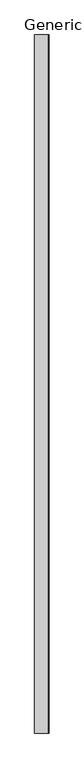
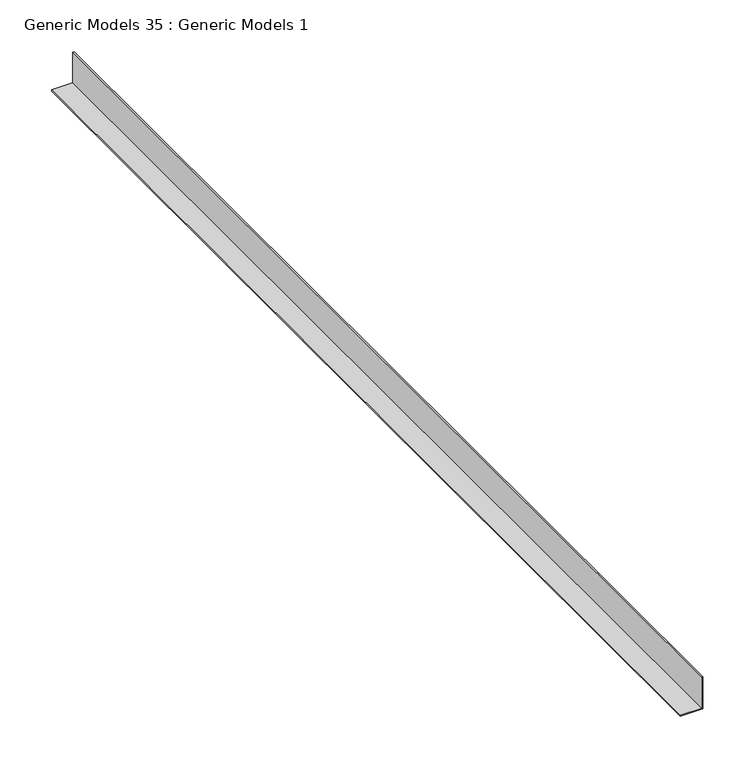
"""IFC4 building model written with IfcOpenShell, lengths in millimetres: proxy geometry, Generic Models 35 : Generic Models 1."""

from ifc_helpers import new_model, si_unit, frame, origin, place, context, project, spatial, polyline, outline, extrude, source, transform, mapped, element, save


def generic_models_35_generic_models_1_f99cc74d(model_context):
    return source(origin(), model_context, "Body", "SweptSolid", [
        extrude(outline(polyline([(2277.1204978, 49676.05), (2277.1204978, 49674.4625), (2240.6079978, 49674.4625), (2240.6079978, 49650.65), (2239.0204978, 49650.65), (2239.0204978, 49676.05), (2277.1204978, 49676.05)])), frame((0.0, 0.0, 0.0), z_axis=(0.0, 1.0, 0.0), x_axis=(0.0, 0.0, 1.0)), (0.0, 0.0, 1.0), 1219.2),
    ])


if __name__ == "__main__":
    model = new_model("IFC4")
    model_context = context("Model", 3, world=origin())
    ifc_project = project(units=[si_unit("LENGTHUNIT", "METRE", prefix="MILLI")], contexts=[model_context])
    site = spatial("IfcSite", under=ifc_project)
    building = spatial("IfcBuilding", under=site)
    placement = place(None, origin())
    generic_models_35_generic_models_1_shape = generic_models_35_generic_models_1_f99cc74d(model_context)
    element("IfcBuildingElementProxy", 1, Name="Generic Models 35 : Generic Models 1", ObjectType="Generic Models 35 : Generic Models 1", at=placement, inside=building, context=model_context, shape_type="MappedRepresentation", body=[
        mapped(generic_models_35_generic_models_1_shape, transform((0.0, 0.0, 0.0), x_axis=(1.0, 0.0, 0.0), y_axis=(0.0, 1.0, 0.0), z_axis=(0.0, 0.0, 1.0))),
    ])
    save(model, "model.ifc")

# Revit data of these elements
# Element 1 (IfcBuildingElementProxy, "Generic Models 35 : Generic Models 1")
#   Materials on its faces: "CEILING TRACK AS SCHEDULED"
# Materials
#   "CEILING TRACK AS SCHEDULED": class "Unassigned", colour RGB 210 209 208, transparency 0, Keynote = "M05121300.02", Cost = 0
